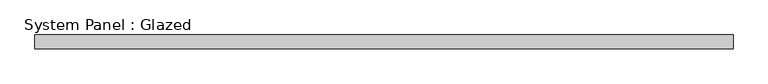
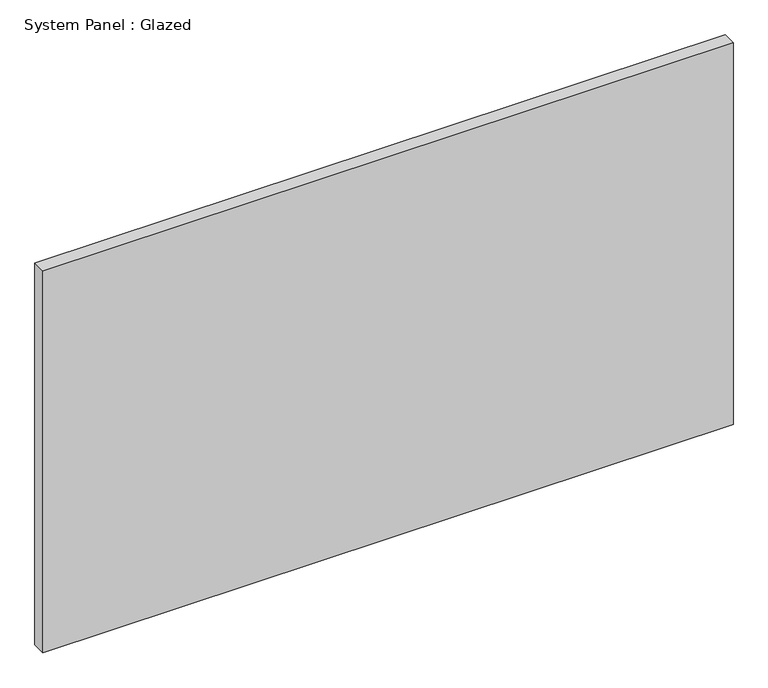
"""IFC4 building model written with IfcOpenShell, lengths in millimetres: plate geometry, System Panel : Glazed."""

from ifc_helpers import new_model, si_unit, origin, origin_with_axes, place, context, project, spatial, polyline, outline, extrude, source, transform, mapped, element, save


def system_panel_glazed_8692f37a(model_context):
    return source(origin(), model_context, "Body", "SweptSolid", [
        extrude(outline(polyline([(620.0000001, 24.5), (-620.0000001, 24.5), (-620.0000001, 49.5), (620.0000001, 49.5), (620.0000001, 24.5)])), origin_with_axes(), (0.0, 0.0, 1.0), 725.0),
    ])


if __name__ == "__main__":
    model = new_model("IFC4")
    model_context = context("Model", 3, world=origin())
    ifc_project = project(units=[si_unit("LENGTHUNIT", "METRE", prefix="MILLI")], contexts=[model_context])
    site = spatial("IfcSite", under=ifc_project)
    building = spatial("IfcBuilding", under=site)
    placement = place(None, origin())
    system_panel_glazed_shape = system_panel_glazed_8692f37a(model_context)
    element("IfcPlate", 1, ObjectType="System Panel : Glazed", at=placement, inside=building, context=model_context, shape_type="MappedRepresentation", body=[
        mapped(system_panel_glazed_shape, transform((0.0, 0.0, 0.0), x_axis=(1.0, 0.0, 0.0), y_axis=(0.0, 1.0, 0.0), z_axis=(0.0, 0.0, 1.0))),
    ])
    save(model, "model.ifc")

# Revit data of these elements
# Type "System Panel : Glazed"
#   Construction Type Id = "GSP4R"
#   Analytic Construction = "1/8 in Pilkington single glazing"
#   Visual Light Transmittance = 0.9
#   Solar Heat Gain Coefficient = 0.86
#   Heat Transfer Coefficient (U) = 6.7069 W/(m²·K)
#   Define Thermal Properties by = 1
# Element 1 (IfcPlate, "System Panel : Glazed")
#   Materials on its faces: "Glass"
# Materials
#   "Glass": class "Glass", colour RGB 0 128 192, transparency 0.9, Description = "Soda Lime Glass", Cost = 0
